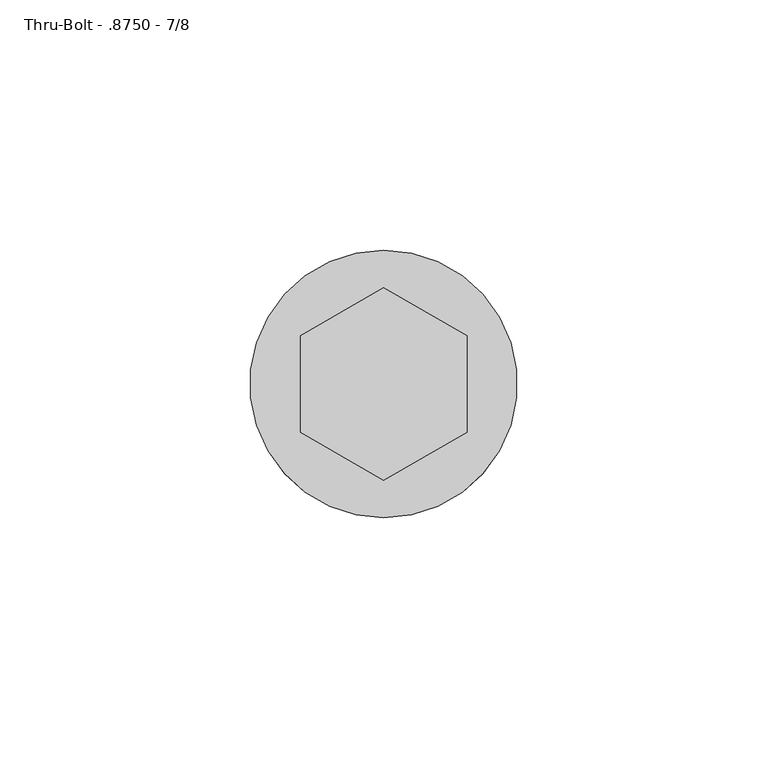
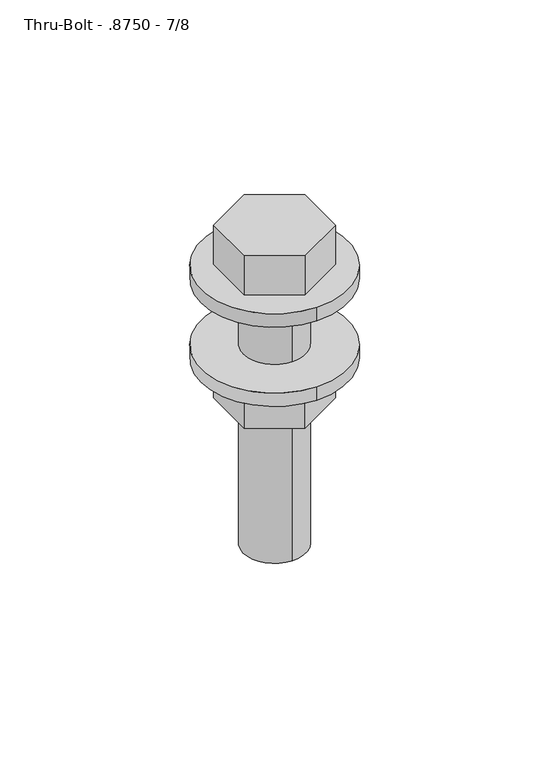
"""IFC4 building model written with IfcOpenShell, lengths in millimetres: fastener geometry, 060523 - W_P_C - Fastenings - Generic : Thru-Bolt - .8750 - 7/8."""

from ifc_helpers import new_model, si_unit, point, frame, origin, origin_with_axes, origin_2d, place, context, project, spatial, polyline, circle_curve, trimmed, segment, composite_curve, outline, extrude, source, transform, mapped, element, save


def thru_bolt_8750_7_8_94ead554(model_context):
    return source(origin(), model_context, "Body", "SweptSolid", [
        extrude(outline(composite_curve([segment(trimmed(circle_curve(origin_2d(), 26.7394531), [point((0.0, 26.7394531))], [point((0.0, -26.7394531))], False, "CARTESIAN"), True, "CONTINUOUS"), segment(trimmed(circle_curve(origin_2d(), 26.7394531), [point((0.0, -26.7394531))], [point((0.0, 26.7394531))], False, "CARTESIAN"), True, "CONTINUOUS")], self_intersect=False)), origin_with_axes(), (0.0, 0.0, 1.0), 5.1263021),
        extrude(outline(composite_curve([segment(trimmed(circle_curve(origin_2d(), 26.7394531), [point((0.0, 26.7394531))], [point((0.0, -26.7394531))], False, "CARTESIAN"), True, "CONTINUOUS"), segment(trimmed(circle_curve(origin_2d(), 26.7394531), [point((0.0, -26.7394531))], [point((0.0, 26.7394531))], False, "CARTESIAN"), True, "CONTINUOUS")], self_intersect=False)), frame((0.0, 0.0, -30.5263021), z_axis=(0.0, 0.0, 1.0), x_axis=(1.0, 0.0, 0.0)), (0.0, 0.0, 1.0), 5.1263021),
        extrude(outline(polyline([(-16.66875, -9.6237073), (-16.66875, 9.6237073), (0.0, 19.2474146), (16.66875, 9.6237073), (16.66875, -9.6237073), (0.0, -19.2474146), (-16.66875, -9.6237073)])), frame((0.0, 0.0, -45.9052083), z_axis=(0.0, 0.0, 1.0), x_axis=(1.0, 0.0, 0.0)), (0.0, 0.0, 1.0), 15.3789062),
        extrude(outline(polyline([(-16.66875, 9.6237073), (0.0, 19.2474146), (16.66875, 9.6237073), (16.66875, -9.6237073), (0.0, -19.2474146), (-16.66875, -9.6237073), (-16.66875, 9.6237073)])), frame((0.0, 0.0, 5.1263021), z_axis=(0.0, 0.0, 1.0), x_axis=(1.0, 0.0, 0.0)), (0.0, 0.0, 1.0), 15.3789062),
        extrude(outline(composite_curve([segment(trimmed(circle_curve(origin_2d(), 11.3605469), [point((0.0, -11.3605469))], [point((0.0, 11.3605469))], False, "CARTESIAN"), True, "CONTINUOUS"), segment(trimmed(circle_curve(origin_2d(), 11.3605469), [point((0.0, 11.3605469))], [point((0.0, -11.3605469))], False, "CARTESIAN"), True, "CONTINUOUS")], self_intersect=False)), frame((0.0, 0.0, -101.6), z_axis=(0.0, 0.0, 1.0), x_axis=(1.0, 0.0, 0.0)), (0.0, 0.0, 1.0), 106.7263021),
    ])


if __name__ == "__main__":
    model = new_model("IFC4")
    model_context = context("Model", 3, world=origin())
    ifc_project = project(units=[si_unit("LENGTHUNIT", "METRE", prefix="MILLI")], contexts=[model_context])
    site = spatial("IfcSite", under=ifc_project)
    building = spatial("IfcBuilding", under=site)
    placement = place(None, origin())
    thru_bolt_8750_7_8_shape = thru_bolt_8750_7_8_94ead554(model_context)
    element("IfcFastener", 1, ObjectType="060523 - W_P_C - Fastenings - Generic : Thru-Bolt - .8750 - 7/8", at=placement, inside=building, context=model_context, shape_type="MappedRepresentation", body=[
        mapped(thru_bolt_8750_7_8_shape, transform((0.0, 0.0, 0.0), x_axis=(1.0, 0.0, 0.0), y_axis=(0.0, 1.0, 0.0), z_axis=(0.0, 0.0, 1.0))),
    ])
    save(model, "model.ifc")

# Revit data of these elements
# Type "060523 - W_P_C - Fastenings - Generic : Thru-Bolt - .8750 - 7/8"
#   Washer_Thickness = 0' - 0.20182"
#   Washer Radius = 0' - 1.05273"
#   Washer Offset - Head = 0' - 0.20182"
#   Washer Offset = 0' - 0.20182"
#   Thickness_of_Substrate [instance default] = 0' - 1"
#   Side = 0' - 0.75879"
#   Radius = 0' - 0.44727"
#   Length [instance default] = 0' - 4"
#   Head Size = 0' - 1 5/16"
#   Head Radius = 0' - 0 21/32"
#   Head Height = 0' - 0 155/256"
#   Double Diameter = 0' - 1 101/128"
#   Diameter = 0' - 0 229/256"
#   Default Elevation = 4' - 0"
#   Washer_Nut_Visibility = yes
#   Washer_Head_Visibility = yes
#   Round_Head_Visibility = no
#   Point Visibility = no
#   Nut_Visibility = yes
#   Hex_Head_Visiblilty = yes
#   Washer Material = none
#   Bolt Material (Size) = AT SILL - FASTENER AT 24" O.C.
# Element 1 (IfcFastener, "060523 - W_P_C - Fastenings - Generic : Thru-Bolt - .8750 - 7/8")
#   Materials on its faces: "AT SILL - FASTENER AT 24\" O.C."
# Materials
#   "AT SILL - FASTENER AT 24\" O.C.": class "Generic", colour RGB 120 120 120, transparency 0, Cost = 0
